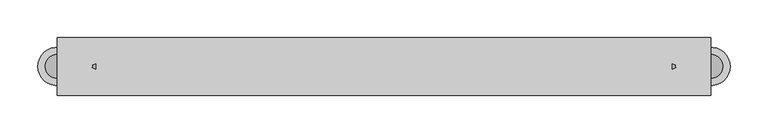
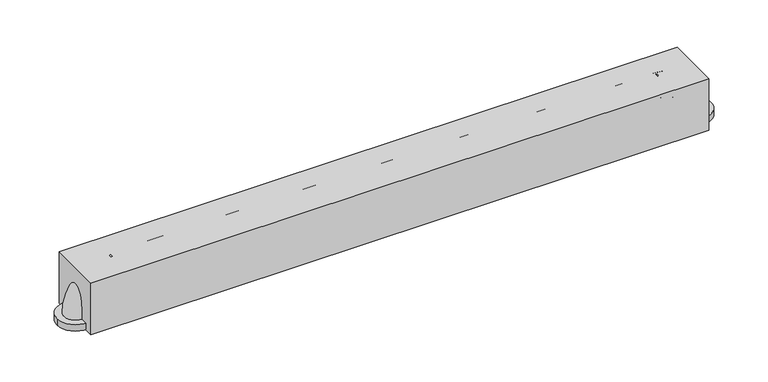
"""IFC4 building model written with IfcOpenShell, lengths in millimetres: proxy geometry, A5109 - Grab Bar, 1.25 in Dia, SS, 2 Wall, W-C Accessible : A5109 - Grab Bar, 1.25 in Dia, SS, 2 Wall, W-C Accessible."""

import ifcopenshell
import ifcopenshell.guid

model = None  # the IFC model being written
_history = None  # IfcOwnerHistory: only IFC2X3 demands one
_inside = {}  # id of a spatial element -> (the spatial element, [elements in it])
_under = {}  # id of a project, library or spatial element -> (it, [spatial elements below it])
_declared = {}  # id of a project -> (the project, [libraries it declares])
_typed = {}  # id of a type object -> (the type object, [elements of that type])
_made_of = {}  # id of a material, layer set ... -> (it, [elements and type objects made of it])


def new_model(schema):
    """Start an empty IFC model of exactly this schema.

    Asked for "IFC4X3", IfcOpenShell would pick the latest addendum, in which some entities
    have other attributes; the version numbers below select the first issue.
    IFC2X3 requires an IfcOwnerHistory on every rooted entity: one is made here for all.
    """
    global model, _history
    if schema == "IFC4X3":
        model = ifcopenshell.file(schema_version=(4, 3, 0, 0))
    else:
        model = ifcopenshell.file(schema=schema)
    _inside.clear()
    _under.clear()
    _declared.clear()
    _typed.clear()
    _made_of.clear()
    _history = None
    if model.schema == "IFC2X3":
        org = make("IfcOrganization", Name="unknown")
        user = make(
            "IfcPersonAndOrganization",
            ThePerson=make("IfcPerson", FamilyName="unknown"),
            TheOrganization=org,
        )
        app = make(
            "IfcApplication",
            ApplicationDeveloper=org,
            Version="unknown",
            ApplicationFullName="unknown",
            ApplicationIdentifier="unknown",
        )
        _history = make(
            "IfcOwnerHistory",
            OwningUser=user,
            OwningApplication=app,
            ChangeAction="ADDED",
            CreationDate=0,
        )
    return model


def make(cls, **values):
    """One entity of the class cls with the attributes given. An attribute that is None is left unset."""
    return model.create_entity(
        cls, **{name: value for name, value in values.items() if value is not None}
    )


def rooted(cls, **values):
    """An entity with a GlobalId (a new one), such as an element, a storey or a relation."""
    return make(cls, GlobalId=ifcopenshell.guid.new(), OwnerHistory=_history, **values)


def si_unit(unit_type, name, prefix=None):
    """IfcSIUnit, for example si_unit("LENGTHUNIT", "METRE", prefix="MILLI")."""
    return make("IfcSIUnit", UnitType=unit_type, Prefix=prefix, Name=name)


def assignment(units):
    """IfcUnitAssignment: the units of a project."""
    return None if units is None else make("IfcUnitAssignment", Units=units)


def point(xyz):
    """IfcCartesianPoint."""
    return None if xyz is None else make("IfcCartesianPoint", Coordinates=xyz)


def direction(xyz):
    """IfcDirection."""
    return None if xyz is None else make("IfcDirection", DirectionRatios=xyz)


def frame(location, z_axis=None, x_axis=None):
    """IfcAxis2Placement3D, a coordinate frame: its origin and axes. An axis left out is left unset."""
    return make(
        "IfcAxis2Placement3D",
        Location=point(location),
        Axis=direction(z_axis),
        RefDirection=direction(x_axis),
    )


def frame_2d(location, x_axis=None):
    """IfcAxis2Placement2D, a coordinate frame in the plane: its origin and x axis."""
    return make(
        "IfcAxis2Placement2D", Location=point(location), RefDirection=direction(x_axis)
    )


def origin():
    """The frame at (0, 0, 0) with its axes left unset."""
    return frame((0.0, 0.0, 0.0))


def origin_with_axes():
    """The frame at (0, 0, 0) with the z axis (0, 0, 1) and the x axis (1, 0, 0) written out."""
    return frame((0.0, 0.0, 0.0), z_axis=(0.0, 0.0, 1.0), x_axis=(1.0, 0.0, 0.0))


def place(relative_to, where):
    """IfcLocalPlacement: puts the frame where relative to a parent placement (None: the world)."""
    return make(
        "IfcLocalPlacement", PlacementRelTo=relative_to, RelativePlacement=where
    )


def context(
    kind, dimensions, precision=None, world=None, true_north=None, identifier=None
):
    """IfcGeometricRepresentationContext, for example the 3D "Model" context."""
    return make(
        "IfcGeometricRepresentationContext",
        ContextIdentifier=identifier,
        ContextType=kind,
        CoordinateSpaceDimension=dimensions,
        Precision=precision,
        WorldCoordinateSystem=world,
        TrueNorth=true_north,
    )


def project(units=None, contexts=None):
    """IfcProject with its units and contexts."""
    return rooted(
        "IfcProject",
        Name="project",
        RepresentationContexts=contexts,
        UnitsInContext=assignment(units),
    )


def spatial(cls, under=None, at=None, **own):
    """A site, building, storey or space (cls), placed at a placement, below another one or the project."""
    s = rooted(cls, ObjectPlacement=at, **own)
    if under is not None:
        _under.setdefault(under.id(), (under, []))[1].append(s)
    return s


def polyline(points):
    """IfcPolyline through the points."""
    return make("IfcPolyline", Points=[point(p) for p in points])


def circle_curve(where, radius):
    """IfcCircle in the frame where."""
    return make("IfcCircle", Position=where, Radius=radius)


def ellipse_curve(where, semi_axis1, semi_axis2):
    """IfcEllipse in the frame where."""
    return make(
        "IfcEllipse", Position=where, SemiAxis1=semi_axis1, SemiAxis2=semi_axis2
    )


def trimmed(basis, trim1, trim2, sense, master):
    """IfcTrimmedCurve: the piece of a basis curve between two trims."""
    return make(
        "IfcTrimmedCurve",
        BasisCurve=basis,
        Trim1=trim1,
        Trim2=trim2,
        SenseAgreement=sense,
        MasterRepresentation=master,
    )


def segment(curve, same_sense, transition):
    """IfcCompositeCurveSegment."""
    return make(
        "IfcCompositeCurveSegment",
        Transition=transition,
        SameSense=same_sense,
        ParentCurve=curve,
    )


def composite_curve(segments, self_intersect=None):
    """IfcCompositeCurve: segments joined end to end."""
    return make("IfcCompositeCurve", Segments=segments, SelfIntersect=self_intersect)


def outline(outer, holes=None, kind="AREA"):
    """IfcArbitraryClosedProfileDef: a profile drawn as a closed curve; with holes, ...WithVoids."""
    if holes is None:
        return make("IfcArbitraryClosedProfileDef", ProfileType=kind, OuterCurve=outer)
    return make(
        "IfcArbitraryProfileDefWithVoids",
        ProfileType=kind,
        OuterCurve=outer,
        InnerCurves=holes,
    )


def extrude(swept, where, along, depth):
    """IfcExtrudedAreaSolid: the profile swept, set in the frame where, extruded along a direction by depth."""
    return make(
        "IfcExtrudedAreaSolid",
        SweptArea=swept,
        Position=where,
        ExtrudedDirection=direction(along),
        Depth=depth,
    )


def shape(context_of_items, identifier, shape_type, items):
    """IfcShapeRepresentation: the items that make up one representation, for example the "Body"."""
    return make(
        "IfcShapeRepresentation",
        ContextOfItems=context_of_items,
        RepresentationIdentifier=identifier,
        RepresentationType=shape_type,
        Items=items,
    )


def source(mapping_origin, context_of_items, identifier, shape_type, items):
    """IfcRepresentationMap: a shape defined once, which mapped items show again and again."""
    return make(
        "IfcRepresentationMap",
        MappingOrigin=mapping_origin,
        MappedRepresentation=shape(context_of_items, identifier, shape_type, items),
    )


def transform(
    local_origin,
    x_axis=None,
    y_axis=None,
    z_axis=None,
    scale=None,
    scale2=None,
    scale3=None,
    uniform=True,
):
    """IfcCartesianTransformationOperator3D, or its non-uniform kind. x_axis, y_axis, z_axis: its Axis1, 2, 3."""
    if uniform:
        return make(
            "IfcCartesianTransformationOperator3D",
            Axis1=direction(x_axis),
            Axis2=direction(y_axis),
            LocalOrigin=point(local_origin),
            Scale=scale,
            Axis3=direction(z_axis),
        )
    return make(
        "IfcCartesianTransformationOperator3DnonUniform",
        Axis1=direction(x_axis),
        Axis2=direction(y_axis),
        LocalOrigin=point(local_origin),
        Scale=scale,
        Axis3=direction(z_axis),
        Scale2=scale2,
        Scale3=scale3,
    )


def mapped(mapping_source, mapping_target):
    """IfcMappedItem: shows the shape of a source again, moved by a transform."""
    return make(
        "IfcMappedItem", MappingSource=mapping_source, MappingTarget=mapping_target
    )


def made_of(thing, what):
    """Note that an element or type object is made of a material, layer set ...; save() writes the relation."""
    if what is not None:
        _made_of.setdefault(what.id(), (what, []))[1].append(thing)
    return thing


def element(
    cls,
    number,
    at=None,
    inside=None,
    cuts=None,
    type_object=None,
    material=None,
    context=None,
    identifier="Body",
    shape_type=None,
    held_by="IfcProductDefinitionShape",
    body=None,
    shapes=None,
    **own,
):
    """One element of the class cls, such as IfcWall. Its Tag is "e" and its number.

    at: its placement. inside: the storey or other place that contains it. cuts: it is an
    opening in that element (IfcRelVoidsElement). A single representation is given by context,
    identifier, shape_type and body (its items); several are given by shapes. held_by: the class
    of the entity that holds the representations. save() writes the other relations.
    """
    e = rooted(cls, Tag="e%d" % number, ObjectPlacement=at, **own)
    if body is not None:
        shapes = [shape(context, identifier, shape_type, body)]
    if shapes is not None:
        e.Representation = make(held_by, Representations=shapes)
    if inside is not None:
        _inside.setdefault(inside.id(), (inside, []))[1].append(e)
    if cuts is not None:
        rooted(
            "IfcRelVoidsElement", RelatingBuildingElement=cuts, RelatedOpeningElement=e
        )
    if type_object is not None:
        _typed.setdefault(type_object.id(), (type_object, []))[1].append(e)
    return made_of(e, material)


def aggregate(whole, parts):
    """IfcRelAggregates: a whole, such as a stair, and the parts it consists of."""
    return rooted("IfcRelAggregates", RelatingObject=whole, RelatedObjects=parts)


def save(model, path):
    """Write the relations noted so far, then the file.

    IfcRelAggregates (storeys below a building ...), IfcRelContainedInSpatialStructure (elements
    in a storey), IfcRelDefinesByType, IfcRelAssociatesMaterial and IfcRelDeclares: one each for
    every whole, place, type object, material and project.
    """
    for whole, parts in _under.values():
        aggregate(whole, parts)
    for where, things in _inside.values():
        rooted(
            "IfcRelContainedInSpatialStructure",
            RelatedElements=things,
            RelatingStructure=where,
        )
    for kind, things in _typed.values():
        rooted("IfcRelDefinesByType", RelatedObjects=things, RelatingType=kind)
    for what, things in _made_of.values():
        rooted("IfcRelAssociatesMaterial", RelatedObjects=things, RelatingMaterial=what)
    for by, libraries in _declared.values():
        rooted("IfcRelDeclares", RelatingContext=by, RelatedDefinitions=libraries)
    model.write(path)


def plane_surface(at):
    """IfcPlane: the flat surface through the origin of the frame at, square to its z axis."""
    return make("IfcPlane", Position=at)


def revolved_surface(curve, axis_point, axis_direction):
    """IfcSurfaceOfRevolution: the curve turned about the line through axis_point along axis_direction."""
    return make(
        "IfcSurfaceOfRevolution",
        SweptCurve=make("IfcArbitraryOpenProfileDef", ProfileType="CURVE", Curve=curve),
        AxisPosition=make("IfcAxis1Placement", Location=point(axis_point), Axis=direction(axis_direction)),
    )


def advanced_brep(points, edges, surfaces, faces):
    """IfcAdvancedBrep: a solid bounded by faces that lie on surfaces and meet in shared edges.

    An edge is (start, end): straight between two places in points (the first is 0);
    or (start, end, curve); or (start, end, curve, False) where it runs against its curve.
    A face is (place in surfaces, loops), or (place, loops, False) where it looks against
    its surface's normal. A loop lists edges by number (the first is 1), with a minus sign
    where the edge is run from its end to its start. The first loop is the outer one.
    """
    corners = [point(p) for p in points]
    vertices = [make("IfcVertexPoint", VertexGeometry=c) for c in corners]
    made = []
    for start, end, *more in edges:
        made.append(
            make(
                "IfcEdgeCurve",
                EdgeStart=vertices[start],
                EdgeEnd=vertices[end],
                EdgeGeometry=more[0] if more else make("IfcPolyline", Points=[corners[start], corners[end]]),
                SameSense=more[1] if len(more) > 1 else True,
            )
        )
    hull = []
    for where, loops, *sense in faces:
        bounds = []
        for j, loop in enumerate(loops):
            ring = [make("IfcOrientedEdge", EdgeElement=made[abs(k) - 1], Orientation=k > 0) for k in loop]
            bounds.append(
                make(
                    "IfcFaceOuterBound" if j == 0 else "IfcFaceBound",
                    Bound=make("IfcEdgeLoop", EdgeList=ring),
                    Orientation=True,
                )
            )
        hull.append(make("IfcAdvancedFace", Bounds=bounds, FaceSurface=surfaces[where], SameSense=sense[0] if sense else True))
    return make("IfcAdvancedBrep", Outer=make("IfcClosedShell", CfsFaces=hull))


def specialty_equipment_42bb13b5(model_context):
    return source(origin(), model_context, "Body", "SolidModel", [
        advanced_brep(
        [(381.0, -15.875, 60.325), (381.0, 15.875, 60.325), (431.8, -15.875, 9.525), (431.8, 15.875, 9.525)],
        [
            (0, 1, circle_curve(frame((381.0, 0.0, 60.325), z_axis=(-1.0, 0.0, 0.0), x_axis=(0.0, 1.0, 0.0)), 15.875)),
            (1, 0, circle_curve(frame((381.0, 0.0, 60.325), z_axis=(-1.0, 0.0, 0.0), x_axis=(0.0, 1.0, 0.0)), 15.875)),
            (2, 3, circle_curve(frame((431.8, 0.0, 9.525), z_axis=(0.0, 0.0, -1.0), x_axis=(0.0, 1.0, 0.0)), 15.875)),
            (3, 2, circle_curve(frame((431.8, 0.0, 9.525), z_axis=(0.0, 0.0, -1.0), x_axis=(0.0, 1.0, 0.0)), 15.875)),
            (3, 1, circle_curve(frame((381.0, 15.875, 9.525), z_axis=(0.0, -1.0, 0.0), x_axis=(0.0, 0.0, 1.0)), 50.8)),
            (0, 2, circle_curve(frame((381.0, -15.875, 9.525), z_axis=(0.0, 1.0, 0.0), x_axis=(0.0, 0.0, 1.0)), 50.8)),
        ],
        [
            plane_surface(frame((381.0, 0.0, 60.325), z_axis=(-1.0, 0.0, 0.0), x_axis=(0.0, 1.0, 0.0))),
            plane_surface(frame((431.8, 0.0, 9.525), z_axis=(0.0, 0.0, -1.0), x_axis=(0.0, 1.0, 0.0))),
            revolved_surface(trimmed(ellipse_curve(frame((381.0, 0.0, 60.325), z_axis=(-1.0, 0.0, 0.0), x_axis=(0.0, 1.0, 0.0)), 15.875, 15.875), [point((381.0, -15.875, 60.325))], [point((381.0, 15.875, 60.325))], True, "CARTESIAN"), (381.0, 0.0, 9.525), (0.0, 1.0, 0.0)),
            revolved_surface(trimmed(ellipse_curve(frame((381.0, 0.0, 60.325), z_axis=(-1.0, 0.0, 0.0), x_axis=(0.0, 1.0, 0.0)), 15.875, 15.875), [point((381.0, 15.875, 60.325))], [point((381.0, -15.875, 60.325))], True, "CARTESIAN"), (381.0, 0.0, 9.525), (0.0, 1.0, 0.0)),
        ],
        [
            (0, [[1, 2]]),
            (1, [[3, 4]]),
            (2, [[5, -1, 6, -4]]),
            (3, [[-6, -2, -5, -3]]),
        ],
    ),
        extrude(outline(composite_curve([segment(trimmed(circle_curve(frame_2d((431.8, 0.0)), 25.4), [point((457.2, 0.0))], [point((406.4, 0.0))], False, "CARTESIAN"), True, "CONTINUOUS"), segment(trimmed(circle_curve(frame_2d((431.8, 0.0)), 25.4), [point((406.4, 0.0))], [point((457.2, 0.0))], False, "CARTESIAN"), True, "CONTINUOUS")], self_intersect=False)), origin_with_axes(), (0.0, 0.0, 1.0), 9.525),
        advanced_brep(
        [(-381.0, -15.875, 60.325), (-381.0, 15.875, 60.325), (-431.8, -15.875, 9.525), (-431.8, 15.875, 9.525)],
        [
            (0, 1, circle_curve(frame((-381.0, 0.0, 60.325), z_axis=(1.0, 0.0, 0.0), x_axis=(0.0, 1.0, 0.0)), 15.875)),
            (1, 0, circle_curve(frame((-381.0, 0.0, 60.325), z_axis=(1.0, 0.0, 0.0), x_axis=(0.0, 1.0, 0.0)), 15.875)),
            (2, 3, circle_curve(frame((-431.8, 0.0, 9.525), z_axis=(0.0, 0.0, -1.0), x_axis=(0.0, 1.0, 0.0)), 15.875)),
            (3, 2, circle_curve(frame((-431.8, 0.0, 9.525), z_axis=(0.0, 0.0, -1.0), x_axis=(0.0, 1.0, 0.0)), 15.875)),
            (2, 0, circle_curve(frame((-381.0, -15.875, 9.525), z_axis=(0.0, 1.0, 0.0), x_axis=(0.0, 0.0, 1.0)), 50.8)),
            (1, 3, circle_curve(frame((-381.0, 15.875, 9.525), z_axis=(0.0, -1.0, 0.0), x_axis=(0.0, 0.0, 1.0)), 50.8)),
        ],
        [
            plane_surface(frame((-381.0, 0.0, 60.325), z_axis=(1.0, 0.0, 0.0), x_axis=(0.0, 1.0, 0.0))),
            plane_surface(frame((-431.8, 0.0, 9.525), z_axis=(0.0, 0.0, -1.0), x_axis=(0.0, 1.0, 0.0))),
            revolved_surface(trimmed(ellipse_curve(frame((-381.0, 0.0, 60.325), z_axis=(-1.0, 0.0, 0.0), x_axis=(0.0, 1.0, 0.0)), 15.875, 15.875), [point((-381.0, -15.875, 60.325))], [point((-381.0, 15.875, 60.325))], True, "CARTESIAN"), (-381.0, 0.0, 9.525), (0.0, 1.0, 0.0)),
            revolved_surface(trimmed(ellipse_curve(frame((-381.0, 0.0, 60.325), z_axis=(-1.0, 0.0, 0.0), x_axis=(0.0, 1.0, 0.0)), 15.875, 15.875), [point((-381.0, 15.875, 60.325))], [point((-381.0, -15.875, 60.325))], True, "CARTESIAN"), (-381.0, 0.0, 9.525), (0.0, 1.0, 0.0)),
        ],
        [
            (0, [[1, 2]]),
            (1, [[3, 4]]),
            (2, [[-3, 5, -2, 6]]),
            (3, [[-4, -6, -1, -5]]),
        ],
    ),
        extrude(outline(composite_curve([segment(trimmed(circle_curve(frame_2d((-431.8, 0.0)), 25.4), [point((-457.2, 0.0))], [point((-406.4, 0.0))], False, "CARTESIAN"), True, "CONTINUOUS"), segment(trimmed(circle_curve(frame_2d((-431.8, 0.0)), 25.4), [point((-406.4, 0.0))], [point((-457.2, 0.0))], False, "CARTESIAN"), True, "CONTINUOUS")], self_intersect=False)), origin_with_axes(), (0.0, 0.0, 1.0), 9.525),
        extrude(outline(polyline([(431.8, 38.1), (431.8, -38.1), (-431.8, -38.1), (-431.8, 38.1), (431.8, 38.1)])), origin_with_axes(), (0.0, 0.0, 1.0), 76.2),
        extrude(outline(composite_curve([segment(trimmed(circle_curve(frame_2d((0.0, 60.325)), 15.875), [point((15.875, 60.325))], [point((-15.875, 60.325))], False, "CARTESIAN"), True, "CONTINUOUS"), segment(trimmed(circle_curve(frame_2d((0.0, 60.325)), 15.875), [point((-15.875, 60.325))], [point((15.875, 60.325))], False, "CARTESIAN"), True, "CONTINUOUS")], self_intersect=False)), frame((-381.0, 0.0, 0.0), z_axis=(1.0, 0.0, 0.0), x_axis=(0.0, 1.0, 0.0)), (0.0, 0.0, 1.0), 762.0),
    ])


if __name__ == "__main__":
    model = new_model("IFC4")
    model_context = context("Model", 3, world=origin())
    ifc_project = project(units=[si_unit("LENGTHUNIT", "METRE", prefix="MILLI")], contexts=[model_context])
    site = spatial("IfcSite", under=ifc_project)
    building = spatial("IfcBuilding", under=site)
    placement = place(None, origin())
    specialty_equipment_shape = specialty_equipment_42bb13b5(model_context)
    element("IfcBuildingElementProxy", 1, Name="A5109 - Grab Bar, 1.25 in Dia, SS, 2 Wall, W-C Accessible : A5109 - Grab Bar, 1.25 in Dia, SS, 2 Wall, W-C Accessible", ObjectType="A5109 - Grab Bar, 1.25 in Dia, SS, 2 Wall, W-C Accessible : A5109 - Grab Bar, 1.25 in Dia, SS, 2 Wall, W-C Accessible", at=placement, inside=building, context=model_context, shape_type="MappedRepresentation", body=[
        mapped(specialty_equipment_shape, transform((0.0, 0.0, 0.0), x_axis=(1.0, 0.0, 0.0), y_axis=(0.0, 1.0, 0.0), z_axis=(0.0, 0.0, 1.0))),
    ])
    save(model, "model.ifc")

# Revit data of these elements
# Type "A5109 - Grab Bar, 1.25 in Dia, SS, 2 Wall, W-C Accessible : A5109 - Grab Bar, 1.25 in Dia, SS, 2 Wall, W-C Accessible"
#   Watts2 = "0"
#   Watts1 = "0"
#   Unit_Issue = "EA"
#   UTIL_6_Misc = "-"
#   UTIL_5_NonMedGas = "-"
#   UTIL_4_MiscGas = "-"
#   UTIL_3_MedGas = "-"
#   UTIL_2_Elec = "-"
#   UTIL_1_WaterDrain = "-"
#   Nomenclature = "Grab Bar, 1-1/4\" Dia., SS, 2 Wall, W/C Accessible"
#   NSN = "6530"
#   Location [instance default] = ""
#   JSN = "A5109"
#   Fund_Source_VA = "-"
#   Fund_Source_Navy = "-"
#   Fund_Source_Army = "-"
#   Fund_Source_AF = "-"
#   ELEC_Volts2 = "0"
#   ELEC_Volts1 = "0"
#   ELEC_Phase2 = "0"
#   ELEC_Phase1 = "0"
#   ELEC_HertzSwitch = "0"
#   ELEC_HertzDependent = "0"
#   ELEC_Hertz = "0"
#   ELEC_Amps2 = "0"
#   ELEC_Amps1 = "0"
#   DetailDescription = "A 1-1/4\" diameter, satin finish stainless steel, peened gripping surface, 2 wall toilet stall/ room, grab bar with concealed mounting flanges.  Snap over flanges are provided to conceal mounting screws. A selection of mounting kits and concealed anchor devices are available from the manufacturers for different types of installations. Grab bar shall comply with barrier-free accessibility guidelines for structural strength. For typical water closet applications in toilet stalls and rooms where ADA (American''s With Disabilities Act) requirements must be met."
#   CAT_VA = "A"
#   CAT_Navy = "A"
#   CAT_IHS = "-"
#   CAT_Army = "A"
#   CAT_AF = "A"
#   BTUperhour = "0"
#   Weight_IP = 7
#   Default Elevation = 2' - 9"
#   DIM_Width_IP = 4' - 9"
#   DIM_Height_IP = 0' - 3"
#   DIM_Depth_IP = 0' - 3"
#   CustomLength [instance default] = 2' - 0"
# Element 1 (IfcBuildingElementProxy, "A5109 - Grab Bar, 1.25 in Dia, SS, 2 Wall, W-C Accessible : A5109 - Grab Bar, 1.25 in Dia, SS, 2 Wall, W-C Accessible")
#   Location = "TLTS2"
#   CustomLength = 2' - 10"
#   Materials on its faces: "EquipSpace"
# Materials
#   "EquipSpace": class "Unassigned", colour RGB 221 217 195, transparency 0.5
